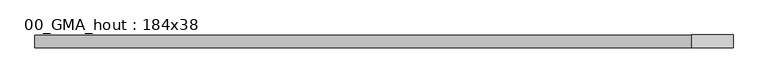
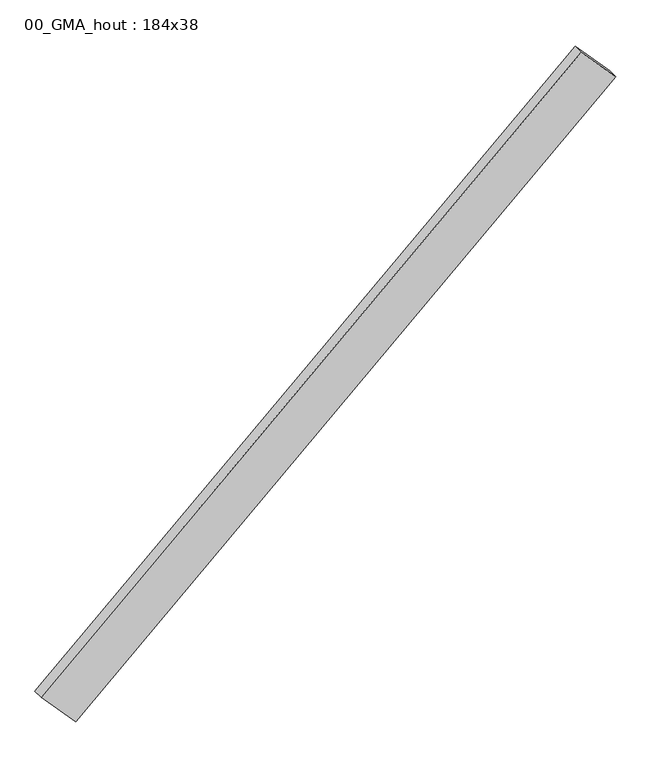
"""IFC4 building model written with IfcOpenShell, lengths in millimetres: proxy geometry, 00_GMA_hout : 184x38."""

from ifc_helpers import new_model, si_unit, frame, origin, place, context, project, spatial, polyline, outline, extrude, source, transform, mapped, element, save


def proxy_00_gma_hout_184x38_d01dc138(model_context):
    return source(origin(), model_context, "Body", "SweptSolid", [
        extrude(outline(polyline([(-19.0, 0.0), (19.0, 0.0), (19.0, -2617.0000001), (-19.0, -2617.0000001), (-19.0, 0.0)])), frame((-400.2270235, -19.0, -613.6855812), z_axis=(-0.67357883778224, 0.0, 0.7391153829355244), x_axis=(0.0, 1.0, 0.0)), (0.0, 0.0, 1.0), 184.0),
    ])


if __name__ == "__main__":
    model = new_model("IFC4")
    model_context = context("Model", 3, world=origin())
    ifc_project = project(units=[si_unit("LENGTHUNIT", "METRE", prefix="MILLI")], contexts=[model_context])
    site = spatial("IfcSite", under=ifc_project)
    building = spatial("IfcBuilding", under=site)
    placement = place(None, origin())
    proxy_00_gma_hout_184x38_shape = proxy_00_gma_hout_184x38_d01dc138(model_context)
    element("IfcBuildingElementProxy", 1, Name="00_GMA_hout : 184x38", ObjectType="00_GMA_hout : 184x38", at=placement, inside=building, context=model_context, shape_type="MappedRepresentation", body=[
        mapped(proxy_00_gma_hout_184x38_shape, transform((0.0, 0.0, 0.0), x_axis=(1.0, 0.0, 0.0), y_axis=(0.0, 1.0, 0.0), z_axis=(0.0, 0.0, 1.0))),
    ])
    save(model, "model.ifc")

# Revit data of these elements
# Type "00_GMA_hout : 184x38"
#   lengte [instance default] = 1198.641 mm
#   h = 38 mm
#   b = 184 mm
#   materiaal = 00_hout_vuren_generiek
#   PositionProfile [instance default] = 00_GMP_rectangle : TopLeft
#   Default Elevation = 0
# Element 1 (IfcBuildingElementProxy, "00_GMA_hout : 184x38")
#   lengte = 2617 mm
#   PositionProfile = 00_GMP_rectangle : BottomRight
#   Materials on its faces: "00_hout_vuren_generiek"
# Materials
#   "00_hout_vuren_generiek": class "Wood", colour RGB 255 128 0, transparency 0, Manufacturer = "RevitGG", URL = "www.revitgg.nl", Description = "Hout, vuren, generiek", Cost = 0
